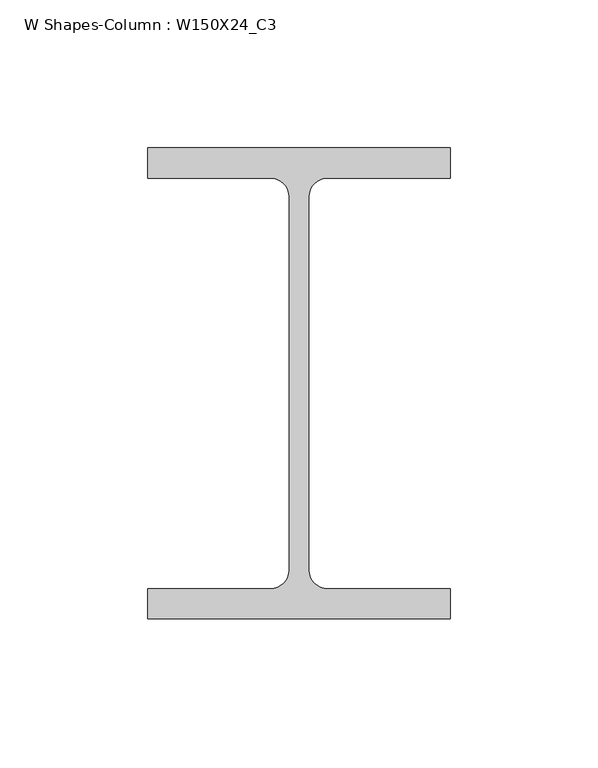
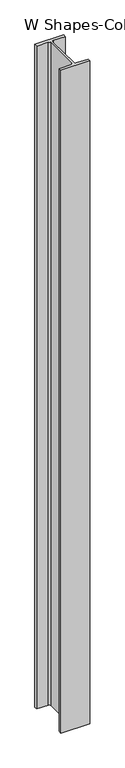
"""IFC4 building model written with IfcOpenShell, lengths in millimetres: column geometry, W Shapes-Column : W150X24_C3."""

from ifc_helpers import new_model, si_unit, point, frame, frame_2d, origin, place, context, project, spatial, polyline, circle_curve, trimmed, segment, composite_curve, outline, extrude, source, transform, mapped, element, save


def w_shapes_column_w150x24_c3_edd9397a(model_context):
    return source(origin(), model_context, "Body", "SweptSolid", [
        extrude(outline(composite_curve([segment(polyline([(51.181, 79.756), (51.181, 69.469), (9.652, 69.469)]), True, "CONTINUOUS"), segment(trimmed(circle_curve(frame_2d((9.652, 63.119)), 6.35), [point((9.652, 69.469))], [point((3.302, 63.119))], True, "CARTESIAN"), True, "CONTINUOUS"), segment(polyline([(3.302, 63.119), (3.302, -63.119)]), True, "CONTINUOUS"), segment(trimmed(circle_curve(frame_2d((9.652, -63.119)), 6.35), [point((3.302, -63.119))], [point((9.652, -69.469))], True, "CARTESIAN"), True, "CONTINUOUS"), segment(polyline([(9.652, -69.469), (51.181, -69.469), (51.181, -79.756), (-51.181, -79.756), (-51.181, -69.469), (-9.652, -69.469)]), True, "CONTINUOUS"), segment(trimmed(circle_curve(frame_2d((-9.652, -63.119)), 6.35), [point((-9.652, -69.469))], [point((-3.302, -63.119))], True, "CARTESIAN"), True, "CONTINUOUS"), segment(polyline([(-3.302, -63.119), (-3.302, 63.119)]), True, "CONTINUOUS"), segment(trimmed(circle_curve(frame_2d((-9.652, 63.119)), 6.35), [point((-3.302, 63.119))], [point((-9.652, 69.469))], True, "CARTESIAN"), True, "CONTINUOUS"), segment(polyline([(-9.652, 69.469), (-51.181, 69.469), (-51.181, 79.756), (51.181, 79.756)]), True, "CONTINUOUS")], self_intersect=False)), frame((0.0, 0.0, 9566.0), z_axis=(0.0, 0.0, 1.0), x_axis=(1.0, 0.0, 0.0)), (0.0, 0.0, 1.0), 2484.0),
    ])


if __name__ == "__main__":
    model = new_model("IFC4")
    model_context = context("Model", 3, world=origin())
    ifc_project = project(units=[si_unit("LENGTHUNIT", "METRE", prefix="MILLI")], contexts=[model_context])
    site = spatial("IfcSite", under=ifc_project)
    building = spatial("IfcBuilding", under=site)
    placement = place(None, origin())
    w_shapes_column_w150x24_c3_shape = w_shapes_column_w150x24_c3_edd9397a(model_context)
    element("IfcColumn", 1, ObjectType="W Shapes-Column : W150X24_C3", at=placement, inside=building, context=model_context, shape_type="MappedRepresentation", body=[
        mapped(w_shapes_column_w150x24_c3_shape, transform((0.0, 0.0, 0.0), x_axis=(1.0, 0.0, 0.0), y_axis=(0.0, 1.0, 0.0), z_axis=(0.0, 0.0, 1.0))),
    ])
    save(model, "model.ifc")

# Revit data of these elements
# Type "W Shapes-Column : W150X24_C3"
#   Section Name Key = "W6x16"
#   Assembly Code = "B10"
#   Width = 10.2362 cm
#   Web Thickness = 0.6604 cm
#   Web Fillet = 0.635 cm
#   Warping Constant = 10258.1 cm⁶
#   Torsional Moment of Inertia = 9.28196 cm⁴
#   Section Area = 30.5806 cm²
#   Plastic Modulus weak axis = 55.5521 cm³
#   Plastic Modulus strong axis = 191.729 cm³
#   Perimeter = 0.704088 m²/m
#   Nominal Weight = 23.8106 kgf/m
#   Moment of Inertia weak axis = 184.391 cm⁴
#   Moment of Inertia strong axis = 1336.10 cm⁴
#   Height = 15.9512 cm
#   Flange Thickness = 1.0287 cm
#   Elastic Modulus weak axis = 36.0515 cm³
#   Elastic Modulus strong axis = 167.148 cm³
#   Clear Web Height = 19.05 cm
#   Centroid Vertical = 7.9756 cm
#   Centroid Horizontal = 5.1181 cm
#   Bolt Spacing = 5.715 cm
#   Structural Material [instance default] = Steel ASTM A992
#   Principal Axes Angle = 0
# Element 1 (IfcColumn, "W Shapes-Column : W150X24_C3")
#   Structural Material = none
# Materials
#   "Steel ASTM A992": class "Metal", colour RGB 199 199 199, transparency 0, Description = "Structural steel 50ksi", Cost = 0
